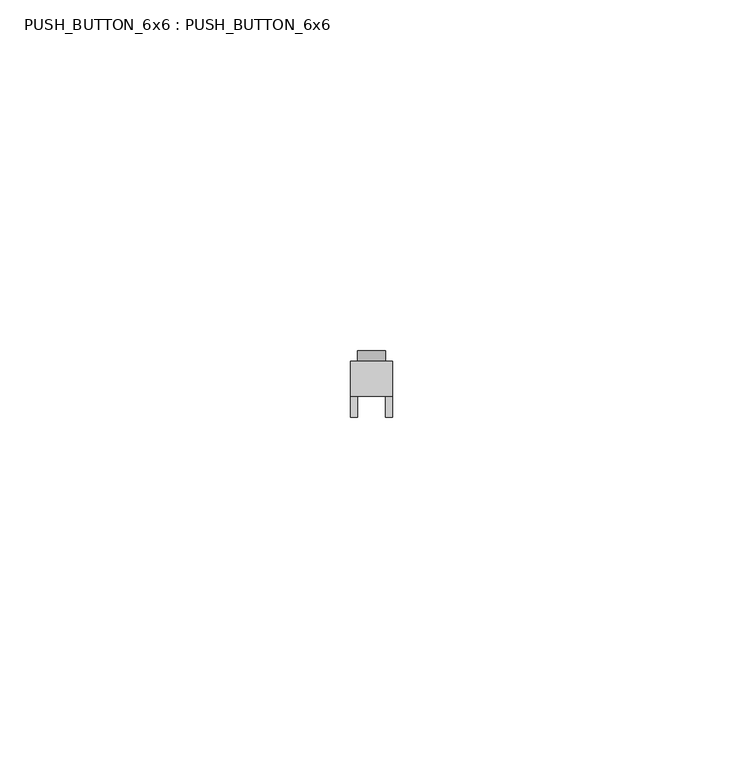
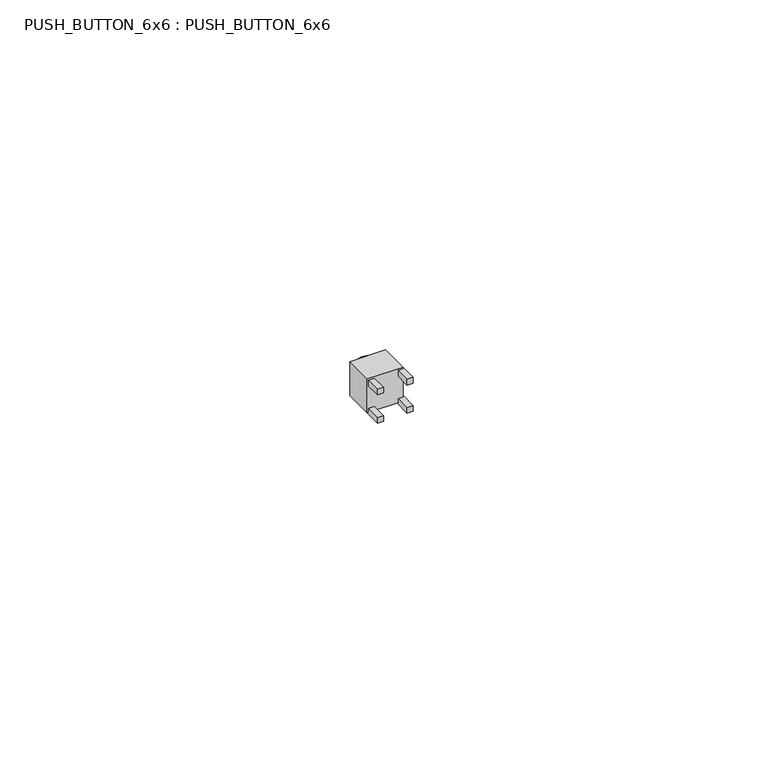
"""IFC4 building model written with IfcOpenShell, lengths in millimetres: furniture geometry, PUSH_BUTTON_6x6 : PUSH_BUTTON_6x6."""

from ifc_helpers import new_model, si_unit, point, frame, frame_2d, origin, origin_with_axes, place, context, project, spatial, polyline, circle_curve, trimmed, segment, composite_curve, outline, extrude, source, transform, mapped, element, save


def push_button_6x6_push_button_6x6_05097e20(model_context):
    return source(origin(), model_context, "Body", "SweptSolid", [
        extrude(outline(polyline([(-3.0, 0.0), (3.0, 0.0), (3.0, -5.0), (-3.0, -5.0), (-3.0, 0.0)])), origin_with_axes(), (0.0, 0.0, 1.0), 6.0),
        extrude(outline(composite_curve([segment(trimmed(circle_curve(frame_2d((3.0, 0.0)), 2.0), [point((3.0, -2.0))], [point((3.0, 2.0))], False, "CARTESIAN"), True, "CONTINUOUS"), segment(trimmed(circle_curve(frame_2d((3.0, 0.0)), 2.0), [point((3.0, 2.0))], [point((3.0, -2.0))], False, "CARTESIAN"), True, "CONTINUOUS")], self_intersect=False)), frame((0.0, 0.0, 0.0), z_axis=(0.0, 1.0, 0.0), x_axis=(0.0, 0.0, 1.0)), (0.0, 0.0, 1.0), 1.5),
        extrude(outline(polyline([(3.0, -5.0), (3.0, -8.0), (2.0, -8.0), (2.0, -5.0), (3.0, -5.0)])), frame((0.0, 0.0, 5.0), z_axis=(0.0, 0.0, 1.0), x_axis=(1.0, 0.0, 0.0)), (0.0, 0.0, 1.0), 1.0),
        extrude(outline(polyline([(-2.0, -5.0), (-2.0, -8.0), (-3.0, -8.0), (-3.0, -5.0), (-2.0, -5.0)])), frame((0.0, 0.0, 5.0), z_axis=(0.0, 0.0, 1.0), x_axis=(1.0, 0.0, 0.0)), (0.0, 0.0, 1.0), 1.0),
        extrude(outline(polyline([(3.0, -5.0), (3.0, -8.0), (2.0, -8.0), (2.0, -5.0), (3.0, -5.0)])), origin_with_axes(), (0.0, 0.0, 1.0), 1.0),
        extrude(outline(polyline([(-2.0, -5.0), (-2.0, -8.0), (-3.0, -8.0), (-3.0, -5.0), (-2.0, -5.0)])), origin_with_axes(), (0.0, 0.0, 1.0), 1.0),
    ])


if __name__ == "__main__":
    model = new_model("IFC4")
    model_context = context("Model", 3, world=origin())
    ifc_project = project(units=[si_unit("LENGTHUNIT", "METRE", prefix="MILLI")], contexts=[model_context])
    site = spatial("IfcSite", under=ifc_project)
    building = spatial("IfcBuilding", under=site)
    placement = place(None, origin())
    push_button_6x6_push_button_6x6_shape = push_button_6x6_push_button_6x6_05097e20(model_context)
    element("IfcFurniture", 1, ObjectType="PUSH_BUTTON_6x6 : PUSH_BUTTON_6x6", at=placement, inside=building, context=model_context, shape_type="MappedRepresentation", body=[
        mapped(push_button_6x6_push_button_6x6_shape, transform((0.0, 0.0, 0.0), x_axis=(1.0, 0.0, 0.0), y_axis=(0.0, 1.0, 0.0), z_axis=(0.0, 0.0, 1.0))),
    ])
    save(model, "model.ifc")

# Revit data of these elements
# Type "PUSH_BUTTON_6x6 : PUSH_BUTTON_6x6"
#   Default Elevation = 0
# Element 1 (IfcFurniture, "PUSH_BUTTON_6x6 : PUSH_BUTTON_6x6")
#   Materials on its faces: ".BOTAO"
# Materials
#   ".BOTAO": class "Vidro", colour RGB 0 255 255, transparency 0.75, Cost = 0
